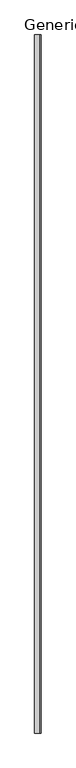
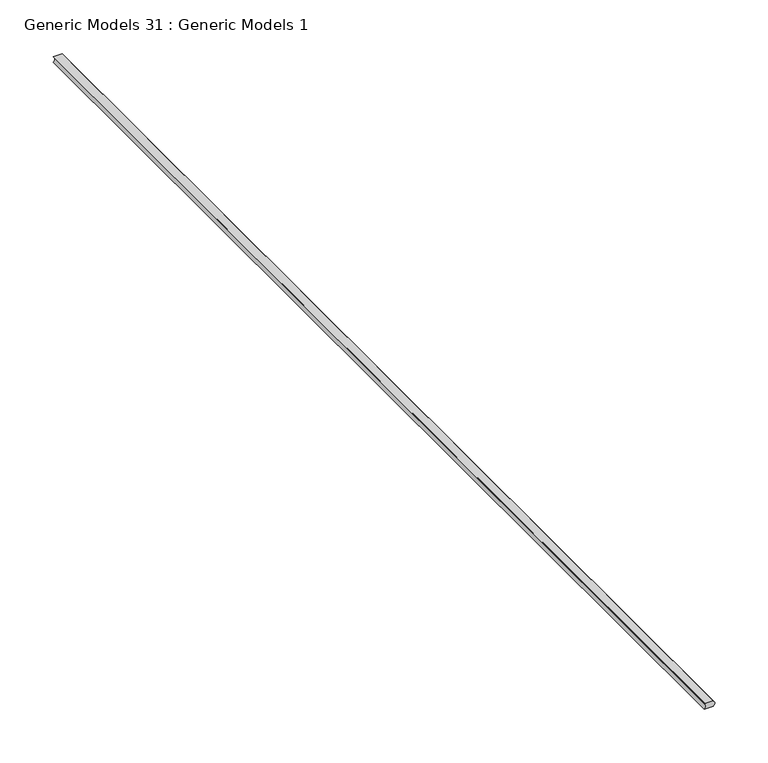
"""IFC4 building model written with IfcOpenShell, lengths in millimetres: proxy geometry, Generic Models 31 : Generic Models 1."""

from ifc_helpers import new_model, si_unit, point, frame, frame_2d, origin, place, context, project, spatial, polyline, circle_curve, trimmed, segment, composite_curve, outline, extrude, source, transform, mapped, element, save


def generic_models_31_generic_models_1_de47f0a2(model_context):
    return source(origin(), model_context, "Body", "SweptSolid", [
        extrude(outline(composite_curve([segment(polyline([(0.0, 48456.85), (0.0, 48466.375)]), True, "CONTINUOUS"), segment(trimmed(circle_curve(frame_2d((3.175, 48463.4602595)), 4.3100275), [point((0.0, 48466.375))], [point((6.35, 48466.375))], False, "CARTESIAN"), True, "CONTINUOUS"), segment(polyline([(6.35, 48466.375), (6.35, 48456.85)]), True, "CONTINUOUS"), segment(trimmed(circle_curve(frame_2d((3.175, 48453.9352595)), 4.3100275), [point((6.35, 48456.85))], [point((0.0, 48456.85))], True, "CARTESIAN"), True, "CONTINUOUS")], self_intersect=False)), frame((0.0, 0.0, 0.0), z_axis=(0.0, 1.0, 0.0), x_axis=(0.0, 0.0, 1.0)), (0.0, 0.0, 1.0), 1219.2),
    ])


if __name__ == "__main__":
    model = new_model("IFC4")
    model_context = context("Model", 3, world=origin())
    ifc_project = project(units=[si_unit("LENGTHUNIT", "METRE", prefix="MILLI")], contexts=[model_context])
    site = spatial("IfcSite", under=ifc_project)
    building = spatial("IfcBuilding", under=site)
    placement = place(None, origin())
    generic_models_31_generic_models_1_shape = generic_models_31_generic_models_1_de47f0a2(model_context)
    element("IfcBuildingElementProxy", 1, Name="Generic Models 31 : Generic Models 1", ObjectType="Generic Models 31 : Generic Models 1", at=placement, inside=building, context=model_context, shape_type="MappedRepresentation", body=[
        mapped(generic_models_31_generic_models_1_shape, transform((0.0, 0.0, 0.0), x_axis=(1.0, 0.0, 0.0), y_axis=(0.0, 1.0, 0.0), z_axis=(0.0, 0.0, 1.0))),
    ])
    save(model, "model.ifc")

# Revit data of these elements
# Element 1 (IfcBuildingElementProxy, "Generic Models 31 : Generic Models 1")
#   Materials on its faces: "ACOUSTICAL SEALANT"
# Materials
#   "ACOUSTICAL SEALANT": class "Unassigned", colour RGB 120 120 120, transparency 0, Cost = 0
